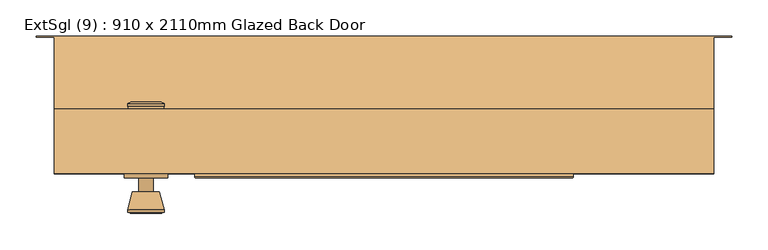
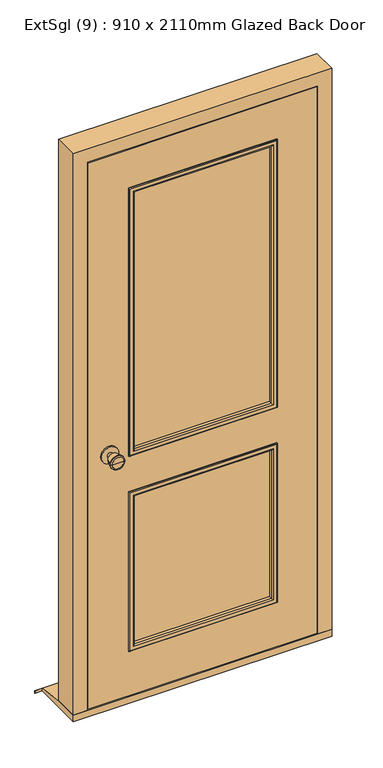
"""IFC4 building model written with IfcOpenShell, lengths in millimetres: door geometry, ExtSgl (9) : 910 x 2110mm Glazed Back Door."""

from ifc_helpers import new_model, si_unit, point, frame, frame_2d, origin, place, context, project, spatial, polyline, circle_curve, ellipse_curve, trimmed, segment, composite_curve, outline, extrude, faceted_brep, source, transform, mapped, element, save
from ifc_brep_helpers import plane_surface, cylinder_surface, revolved_surface, advanced_brep


def extsgl_9_910_x_2110mm_glazed_back_door_d686a627(model_context):
    return source(origin(), model_context, "Body", "SolidModel", [
        advanced_brep(
        [(-328.5, -28.75, 950.0), (-318.5, -28.75, 950.0), (-338.5, -28.75, 950.0), (-308.0241324, -77.75, 950.0), (-328.5, -77.75, 950.0), (-348.9758676, -77.75, 950.0), (-303.5, -75.9221319, 950.0), (-353.5, -75.9221319, 950.0), (-303.5, -72.4584537, 950.0), (-353.5, -72.4584537, 950.0), (-309.863764, -47.75, 950.0), (-347.136236, -47.75, 950.0), (-318.5, -47.75, 950.0), (-338.5, -47.75, 950.0)],
        [
            (0, 1),
            (1, 2, circle_curve(frame((-328.5, -28.75, 950.0), z_axis=(0.0, 1.0, 0.0), x_axis=(-1.0, 0.0, 0.0)), 10.0)),
            (2, 0),
            (2, 1, circle_curve(frame((-328.5, -28.75, 950.0), z_axis=(0.0, 1.0, 0.0), x_axis=(-1.0, 0.0, 0.0)), 10.0)),
            (3, 4),
            (4, 5),
            (5, 3, circle_curve(frame((-328.5, -77.75, 950.0), z_axis=(0.0, -1.0, 0.0), x_axis=(-1.0, 0.0, 0.0)), 20.4758676)),
            (3, 5, circle_curve(frame((-328.5, -77.75, 950.0), z_axis=(0.0, -1.0, 0.0), x_axis=(-1.0, 0.0, 0.0)), 20.4758676)),
            (6, 3),
            (5, 7),
            (7, 6, circle_curve(frame((-328.5, -75.9221319, 950.0), z_axis=(0.0, -1.0, 0.0), x_axis=(-1.0, 0.0, 0.0)), 25.0)),
            (6, 7, circle_curve(frame((-328.5, -75.9221319, 950.0), z_axis=(0.0, -1.0, 0.0), x_axis=(-1.0, 0.0, 0.0)), 25.0)),
            (8, 6),
            (7, 9),
            (9, 8, circle_curve(frame((-328.5, -72.4584537, 950.0), z_axis=(0.0, -1.0, 0.0), x_axis=(-1.0, 0.0, 0.0)), 25.0)),
            (8, 9, circle_curve(frame((-328.5, -72.4584537, 950.0), z_axis=(0.0, -1.0, 0.0), x_axis=(-1.0, 0.0, 0.0)), 25.0)),
            (10, 8),
            (9, 11),
            (11, 10, circle_curve(frame((-328.5, -47.75, 950.0), z_axis=(0.0, -1.0, 0.0), x_axis=(-1.0, 0.0, 0.0)), 18.636236)),
            (10, 11, circle_curve(frame((-328.5, -47.75, 950.0), z_axis=(0.0, -1.0, 0.0), x_axis=(-1.0, 0.0, 0.0)), 18.636236)),
            (12, 10),
            (11, 13),
            (13, 12, circle_curve(frame((-328.5, -47.75, 950.0), z_axis=(0.0, -1.0, 0.0), x_axis=(-1.0, 0.0, 0.0)), 10.0)),
            (12, 13, circle_curve(frame((-328.5, -47.75, 950.0), z_axis=(0.0, -1.0, 0.0), x_axis=(-1.0, 0.0, 0.0)), 10.0)),
            (1, 12),
            (13, 2),
        ],
        [
            plane_surface(frame((-328.5, -28.75, 950.0), z_axis=(0.0, 1.0, 0.0), x_axis=(-1.0, 0.0, 0.0))),
            plane_surface(frame((-328.5, -77.75, 950.0), z_axis=(0.0, -1.0, 0.0), x_axis=(-1.0, 0.0, 0.0))),
            revolved_surface(polyline([(-348.9758676, -77.75, 950.0), (-353.5, -75.9221319, 950.0)]), (-328.5, -28.75, 950.0), (0.0, 1.0, 0.0)),
            cylinder_surface(frame((-328.5, -28.75, 950.0), z_axis=(0.0, 1.0, 0.0), x_axis=(-1.0, 0.0, 0.0)), 25.0),
            revolved_surface(polyline([(-353.5, -72.4584537, 950.0), (-347.136236, -47.75, 950.0)]), (-328.5, -28.75, 950.0), (0.0, 1.0, 0.0)),
            plane_surface(frame((-328.5, -47.75, 950.0), z_axis=(0.0, 1.0, 0.0), x_axis=(-1.0, 0.0, 0.0))),
            cylinder_surface(frame((-328.5, -28.75, 950.0), z_axis=(0.0, 1.0, 0.0), x_axis=(-1.0, 0.0, 0.0)), 10.0),
        ],
        [
            (0, [[1, 2, 3]]),
            (0, [[-3, 4, -1]]),
            (1, [[5, 6, 7]]),
            (1, [[-6, -5, 8]]),
            (2, [[9, -7, 10, 11]]),
            (2, [[-10, -8, -9, 12]]),
            (3, [[13, -11, 14, 15]]),
            (3, [[-14, -12, -13, 16]]),
            (4, [[17, -15, 18, 19]]),
            (4, [[-18, -16, -17, 20]]),
            (5, [[21, -19, 22, 23]]),
            (5, [[-22, -20, -21, 24]]),
            (6, [[25, -23, 26, -2]]),
            (6, [[-26, -24, -25, -4]]),
        ],
    ),
        extrude(outline(composite_curve([segment(trimmed(circle_curve(frame_2d((950.0, -328.5)), 30.0), [point((950.0, -358.5))], [point((950.0, -298.5))], False, "CARTESIAN"), True, "CONTINUOUS"), segment(trimmed(circle_curve(frame_2d((950.0, -328.5)), 30.0), [point((950.0, -298.5))], [point((950.0, -358.5))], False, "CARTESIAN"), True, "CONTINUOUS")], self_intersect=False)), frame((0.0, -28.75, 0.0), z_axis=(0.0, 1.0, 0.0), x_axis=(0.0, 0.0, 1.0)), (0.0, 0.0, 1.0), 6.0),
        advanced_brep(
        [(-328.5, 27.25, 950.0), (-338.5, 27.25, 950.0), (-318.5, 27.25, 950.0), (-308.0241324, 76.25, 950.0), (-348.9758676, 76.25, 950.0), (-328.5, 76.25, 950.0), (-303.5, 74.4221319, 950.0), (-353.5, 74.4221319, 950.0), (-303.5, 70.9584537, 950.0), (-353.5, 70.9584537, 950.0), (-309.863764, 46.25, 950.0), (-347.136236, 46.25, 950.0), (-318.5, 46.25, 950.0), (-338.5, 46.25, 950.0)],
        [
            (0, 1),
            (1, 2, circle_curve(frame((-328.5, 27.25, 950.0), z_axis=(0.0, -1.0, 0.0), x_axis=(-1.0, 0.0, 0.0)), 10.0)),
            (2, 0),
            (2, 1, circle_curve(frame((-328.5, 27.25, 950.0), z_axis=(0.0, -1.0, 0.0), x_axis=(-1.0, 0.0, 0.0)), 10.0)),
            (3, 4, circle_curve(frame((-328.5, 76.25, 950.0), z_axis=(0.0, 1.0, 0.0), x_axis=(-1.0, 0.0, 0.0)), 20.4758676)),
            (4, 5),
            (5, 3),
            (4, 3, circle_curve(frame((-328.5, 76.25, 950.0), z_axis=(0.0, 1.0, 0.0), x_axis=(-1.0, 0.0, 0.0)), 20.4758676)),
            (6, 7, circle_curve(frame((-328.5, 74.4221319, 950.0), z_axis=(0.0, 1.0, 0.0), x_axis=(-1.0, 0.0, 0.0)), 25.0)),
            (7, 4),
            (3, 6),
            (7, 6, circle_curve(frame((-328.5, 74.4221319, 950.0), z_axis=(0.0, 1.0, 0.0), x_axis=(-1.0, 0.0, 0.0)), 25.0)),
            (8, 9, circle_curve(frame((-328.5, 70.9584537, 950.0), z_axis=(0.0, 1.0, 0.0), x_axis=(-1.0, 0.0, 0.0)), 25.0)),
            (9, 7),
            (6, 8),
            (9, 8, circle_curve(frame((-328.5, 70.9584537, 950.0), z_axis=(0.0, 1.0, 0.0), x_axis=(-1.0, 0.0, 0.0)), 25.0)),
            (10, 11, circle_curve(frame((-328.5, 46.25, 950.0), z_axis=(0.0, 1.0, 0.0), x_axis=(-1.0, 0.0, 0.0)), 18.636236)),
            (11, 9),
            (8, 10),
            (11, 10, circle_curve(frame((-328.5, 46.25, 950.0), z_axis=(0.0, 1.0, 0.0), x_axis=(-1.0, 0.0, 0.0)), 18.636236)),
            (12, 13, circle_curve(frame((-328.5, 46.25, 950.0), z_axis=(0.0, 1.0, 0.0), x_axis=(-1.0, 0.0, 0.0)), 10.0)),
            (13, 11),
            (10, 12),
            (13, 12, circle_curve(frame((-328.5, 46.25, 950.0), z_axis=(0.0, 1.0, 0.0), x_axis=(-1.0, 0.0, 0.0)), 10.0)),
            (1, 13),
            (12, 2),
        ],
        [
            plane_surface(frame((-328.5, 27.25, 950.0), z_axis=(0.0, -1.0, 0.0), x_axis=(-1.0, 0.0, 0.0))),
            plane_surface(frame((-328.5, 76.25, 950.0), z_axis=(0.0, 1.0, 0.0), x_axis=(-1.0, 0.0, 0.0))),
            revolved_surface(polyline([(-348.9758676, 76.25, 950.0), (-353.5, 74.4221319, 950.0)]), (-328.5, 27.25, 950.0), (0.0, -1.0, 0.0)),
            cylinder_surface(frame((-328.5, 27.25, 950.0), z_axis=(0.0, -1.0, 0.0), x_axis=(-1.0, 0.0, 0.0)), 25.0),
            revolved_surface(polyline([(-353.5, 70.9584537, 950.0), (-347.136236, 46.25, 950.0)]), (-328.5, 27.25, 950.0), (0.0, -1.0, 0.0)),
            plane_surface(frame((-328.5, 46.25, 950.0), z_axis=(0.0, -1.0, 0.0), x_axis=(-1.0, 0.0, 0.0))),
            cylinder_surface(frame((-328.5, 27.25, 950.0), z_axis=(0.0, -1.0, 0.0), x_axis=(-1.0, 0.0, 0.0)), 10.0),
        ],
        [
            (0, [[1, 2, 3]]),
            (0, [[-3, 4, -1]]),
            (1, [[5, 6, 7]]),
            (1, [[8, -7, -6]]),
            (2, [[9, 10, -5, 11]]),
            (2, [[12, -11, -8, -10]]),
            (3, [[13, 14, -9, 15]]),
            (3, [[16, -15, -12, -14]]),
            (4, [[17, 18, -13, 19]]),
            (4, [[20, -19, -16, -18]]),
            (5, [[21, 22, -17, 23]]),
            (5, [[24, -23, -20, -22]]),
            (6, [[-2, 25, -21, 26]]),
            (6, [[-4, -26, -24, -25]]),
        ],
    ),
        extrude(outline(composite_curve([segment(trimmed(circle_curve(frame_2d((950.0, -328.5)), 30.0), [point((950.0, -358.5))], [point((950.0, -298.5))], False, "CARTESIAN"), True, "CONTINUOUS"), segment(trimmed(circle_curve(frame_2d((950.0, -328.5)), 30.0), [point((950.0, -298.5))], [point((950.0, -358.5))], False, "CARTESIAN"), True, "CONTINUOUS")], self_intersect=False)), frame((0.0, 21.25, 0.0), z_axis=(0.0, 1.0, 0.0), x_axis=(0.0, 0.0, 1.0)), (0.0, 0.0, 1.0), 6.0),
        faceted_brep([(384.5, 66.25, 25.0), (455.0, 66.25, 25.0), (455.0, -22.75, 25.0), (406.5, -22.75, 25.0), (406.5, 24.25, 25.0), (384.5, 24.25, 25.0), (384.5, 66.25, 2039.5), (-384.5, 66.25, 2039.5), (-384.5, 66.25, 25.0), (-455.0, 66.25, 25.0), (-455.0, 66.25, 2110.0), (455.0, 66.25, 2110.0), (455.0, -22.75, 2110.0), (-455.0, -22.75, 2110.0), (-455.0, -22.75, 25.0), (-406.5, -22.75, 25.0), (-406.5, -22.75, 2061.5), (406.5, -22.75, 2061.5), (406.5, 24.25, 2061.5), (-406.5, 24.25, 2061.5), (-406.5, 24.25, 25.0), (-384.5, 24.25, 25.0), (-384.5, 24.25, 2039.5), (384.5, 24.25, 2039.5)], [[[0, 1, 2, 3, 4, 5]], [[1, 0, 6, 7, 8, 9, 10, 11]], [[2, 1, 11, 12]], [[3, 2, 12, 13, 14, 15, 16, 17]], [[4, 3, 17, 18]], [[5, 4, 18, 19, 20, 21, 22, 23]], [[0, 5, 23, 6]], [[7, 22, 21, 8]], [[8, 21, 20, 15, 14, 9]], [[13, 10, 9, 14]], [[19, 16, 15, 20]], [[12, 11, 10, 13]], [[18, 17, 16, 19]], [[6, 23, 22, 7]]]),
        extrude(outline(polyline([(253.5, -12.75), (-253.5, -12.75), (-253.5, 11.25), (253.5, 11.25), (253.5, -12.75)])), frame((0.0, 0.0, 204.0), z_axis=(0.0, 0.0, 1.0), x_axis=(1.0, 0.0, 0.0)), (0.0, 0.0, 1.0), 575.0),
        extrude(outline(polyline([(253.5, -12.75), (-253.5, -12.75), (-253.5, 11.25), (253.5, 11.25), (253.5, -12.75)])), frame((0.0, 0.0, 929.0), z_axis=(0.0, 0.0, 1.0), x_axis=(1.0, 0.0, 0.0)), (0.0, 0.0, 1.0), 979.5),
        faceted_brep([(480.0, 167.25, 0.0), (480.0, 167.25, 9.0947221), (480.0, 166.25, 9.2522001), (480.0, 166.25, 0.0), (-480.0, 167.25, 9.0947221), (-480.0, 167.25, 0.0), (-480.0, 166.25, 0.0), (-480.0, 166.25, 9.2522001), (455.0, 166.25, 0.0), (455.0, -22.75, 0.0), (-455.0, -22.75, 0.0), (-455.0, 166.25, 0.0), (-455.0, 166.25, 9.2522001), (-455.0, 66.25, 25.0), (455.0, 66.25, 25.0), (455.0, 166.25, 9.2522001), (-455.0, -22.75, 25.0), (455.0, -22.75, 25.0)], [[[0, 1, 2, 3]], [[4, 5, 6, 7]], [[5, 0, 3, 8, 9, 10, 11, 6]], [[1, 0, 5, 4]], [[1, 4, 7, 12, 13, 14, 15, 2]], [[13, 16, 17, 14]], [[16, 10, 9, 17]], [[12, 11, 10, 16, 13]], [[11, 12, 7, 6]], [[8, 15, 14, 17, 9]], [[15, 8, 3, 2]]]),
        extrude(outline(polyline([(29.0, 403.5), (2058.5, 403.5), (2058.5, -404.4250294), (29.0, -404.4250294), (29.0, 403.5)]), holes=[polyline([(929.0, -253.5), (1908.5, -253.5), (1908.5, 253.5), (929.0, 253.5), (929.0, -253.5)]), polyline([(204.0, -253.5), (779.0, -253.5), (779.0, 253.5), (204.0, 253.5), (204.0, -253.5)])]), frame((0.0, -22.75, 0.0), z_axis=(0.0, 1.0, 0.0), x_axis=(0.0, 0.0, 1.0)), (0.0, 0.0, 1.0), 44.0),
        advanced_brep(
        [(253.5, -12.75, 779.0), (253.5, -22.75, 779.0), (253.5, -22.75, 204.0), (253.5, -12.75, 204.0), (241.5, -23.75, 767.0), (241.5, -12.75, 767.0), (241.5, -12.75, 216.0), (241.5, -23.75, 216.0), (246.5, -28.75, 772.0), (246.5, -28.75, 211.0), (261.5, -26.75, 787.0), (259.5, -28.75, 785.0), (259.5, -28.75, 198.0), (261.5, -26.75, 196.0), (261.5, -22.75, 787.0), (261.5, -22.75, 196.0), (-253.5, -22.75, 204.0), (-253.5, -12.75, 204.0), (-241.5, -12.75, 216.0), (-241.5, -23.75, 216.0), (-246.5, -28.75, 211.0), (-259.5, -28.75, 198.0), (-261.5, -26.75, 196.0), (-261.5, -22.75, 196.0), (-253.5, -22.75, 779.0), (-253.5, -12.75, 779.0), (-241.5, -12.75, 767.0), (-241.5, -23.75, 767.0), (-246.5, -28.75, 772.0), (-259.5, -28.75, 785.0), (-261.5, -26.75, 787.0), (-261.5, -22.75, 787.0)],
        [
            (0, 1),
            (1, 2),
            (2, 3),
            (3, 0),
            (4, 5),
            (5, 6),
            (6, 7),
            (7, 4),
            (8, 4, ellipse_curve(frame((246.5, -23.75, 772.0), z_axis=(0.7071067811865521, 0.0, -0.7071067811865428), x_axis=(0.7071067811865428, 0.0, 0.7071067811865522)), 7.0710678, 5.0)),
            (7, 9, ellipse_curve(frame((246.5, -23.75, 211.0), z_axis=(0.7071067811865428, 0.0, 0.7071067811865521), x_axis=(-0.707106781186552, 0.0, 0.7071067811865429)), 7.0710678, 5.0)),
            (9, 8),
            (10, 11, ellipse_curve(frame((259.5, -26.75, 785.0), z_axis=(0.7071067811865521, 0.0, -0.7071067811865428), x_axis=(0.7071067811865428, 0.0, 0.7071067811865522)), 2.8284271, 2.0)),
            (11, 12),
            (12, 13, ellipse_curve(frame((259.5, -26.75, 198.0), z_axis=(0.7071067811865428, 0.0, 0.7071067811865521), x_axis=(-0.707106781186552, 0.0, 0.7071067811865429)), 2.8284271, 2.0)),
            (13, 10),
            (14, 10),
            (13, 15),
            (15, 14),
            (2, 16),
            (16, 17),
            (17, 3),
            (6, 18),
            (18, 19),
            (19, 7),
            (19, 20, ellipse_curve(frame((-246.5, -23.75, 211.0), z_axis=(0.7071067811865521, 0.0, -0.7071067811865428), x_axis=(0.7071067811865429, 0.0, 0.707106781186552)), 7.0710678, 5.0)),
            (20, 9),
            (12, 21),
            (21, 22, ellipse_curve(frame((-259.5, -26.75, 198.0), z_axis=(0.7071067811865521, 0.0, -0.7071067811865428), x_axis=(0.7071067811865429, 0.0, 0.707106781186552)), 2.8284271, 2.0)),
            (22, 13),
            (22, 23),
            (23, 15),
            (16, 24),
            (24, 25),
            (25, 17),
            (18, 26),
            (26, 27),
            (27, 19),
            (27, 28, ellipse_curve(frame((-246.5, -23.75, 772.0), z_axis=(-0.7071067811865428, 0.0, -0.7071067811865521), x_axis=(0.707106781186552, 0.0, -0.707106781186543)), 7.0710678, 5.0)),
            (28, 20),
            (21, 29),
            (29, 30, ellipse_curve(frame((-259.5, -26.75, 785.0), z_axis=(-0.7071067811865428, 0.0, -0.7071067811865521), x_axis=(0.707106781186552, 0.0, -0.707106781186543)), 2.8284271, 2.0)),
            (30, 22),
            (30, 31),
            (31, 23),
            (31, 14),
            (1, 24),
            (0, 25),
            (5, 26),
            (4, 27),
            (8, 28),
            (11, 29),
            (10, 30),
        ],
        [
            plane_surface(frame((253.5, -22.75, 779.0), z_axis=(1.0, 0.0, 0.0), x_axis=(0.0, 0.0, -1.0))),
            plane_surface(frame((241.5, -12.75, 767.0), z_axis=(-1.0, 0.0, 0.0), x_axis=(0.0, 0.0, -1.0))),
            cylinder_surface(frame((246.5, -23.75, 779.0), z_axis=(0.0, 0.0, 1.0), x_axis=(1.0, 0.0, 0.0)), 5.0),
            cylinder_surface(frame((259.5, -26.75, 779.0), z_axis=(0.0, 0.0, 1.0), x_axis=(1.0, 0.0, 0.0)), 2.0),
            plane_surface(frame((261.5, -26.75, 787.0), z_axis=(1.0, 0.0, 0.0), x_axis=(0.0, 0.0, -1.0))),
            plane_surface(frame((253.5, -22.75, 204.0), z_axis=(0.0, 0.0, -1.0), x_axis=(-1.0, 0.0, 0.0))),
            plane_surface(frame((241.5, -12.75, 216.0), z_axis=(0.0, 0.0, 1.0), x_axis=(-1.0, 0.0, 0.0))),
            cylinder_surface(frame((253.5, -23.75, 211.0), z_axis=(1.0, 0.0, 0.0), x_axis=(0.0, 0.0, -1.0)), 5.0),
            cylinder_surface(frame((253.5, -26.75, 198.0), z_axis=(1.0, 0.0, 0.0), x_axis=(0.0, 0.0, -1.0)), 2.0),
            plane_surface(frame((261.5, -26.75, 196.0), z_axis=(0.0, 0.0, -1.0), x_axis=(-1.0, 0.0, 0.0))),
            plane_surface(frame((-253.5, -22.75, 204.0), z_axis=(-1.0, 0.0, 0.0), x_axis=(0.0, 0.0, 1.0))),
            plane_surface(frame((-241.5, -12.75, 216.0), z_axis=(1.0, 0.0, 0.0), x_axis=(0.0, 0.0, 1.0))),
            cylinder_surface(frame((-246.5, -23.75, 204.0), z_axis=(0.0, 0.0, -1.0), x_axis=(-1.0, 0.0, 0.0)), 5.0),
            cylinder_surface(frame((-259.5, -26.75, 204.0), z_axis=(0.0, 0.0, -1.0), x_axis=(-1.0, 0.0, 0.0)), 2.0),
            plane_surface(frame((-261.5, -26.75, 196.0), z_axis=(-1.0, 0.0, 0.0), x_axis=(0.0, 0.0, 1.0))),
            plane_surface(frame((-261.5, -22.75, 787.0), z_axis=(0.0, 1.0, 0.0), x_axis=(1.0, 0.0, 0.0))),
            plane_surface(frame((-253.5, -22.75, 779.0), z_axis=(0.0, 0.0, 1.0), x_axis=(1.0, 0.0, 0.0))),
            plane_surface(frame((-253.5, -12.75, 779.0), z_axis=(0.0, 1.0, 0.0), x_axis=(1.0, 0.0, 0.0))),
            plane_surface(frame((-241.5, -12.75, 767.0), z_axis=(0.0, 0.0, -1.0), x_axis=(1.0, 0.0, 0.0))),
            cylinder_surface(frame((-253.5, -23.75, 772.0), z_axis=(-1.0, 0.0, 0.0), x_axis=(0.0, 0.0, 1.0)), 5.0),
            plane_surface(frame((-246.5, -28.75, 772.0), z_axis=(0.0, -1.0, 0.0), x_axis=(1.0, 0.0, 0.0))),
            cylinder_surface(frame((-253.5, -26.75, 785.0), z_axis=(-1.0, 0.0, 0.0), x_axis=(0.0, 0.0, 1.0)), 2.0),
            plane_surface(frame((-261.5, -26.75, 787.0), z_axis=(0.0, 0.0, 1.0), x_axis=(1.0, 0.0, 0.0))),
        ],
        [
            (0, [[1, 2, 3, 4]]),
            (1, [[5, 6, 7, 8]]),
            (2, [[9, -8, 10, 11]]),
            (3, [[12, 13, 14, 15]]),
            (4, [[16, -15, 17, 18]]),
            (5, [[-3, 19, 20, 21]]),
            (6, [[-7, 22, 23, 24]]),
            (7, [[-10, -24, 25, 26]]),
            (8, [[-14, 27, 28, 29]]),
            (9, [[-17, -29, 30, 31]]),
            (10, [[-20, 32, 33, 34]]),
            (11, [[-23, 35, 36, 37]]),
            (12, [[-25, -37, 38, 39]]),
            (13, [[-28, 40, 41, 42]]),
            (14, [[-30, -42, 43, 44]]),
            (15, [[-31, -44, 45, -18], [46, -32, -19, -2]]),
            (16, [[-33, -46, -1, 47]]),
            (17, [[-21, -34, -47, -4], [48, -35, -22, -6]]),
            (18, [[-36, -48, -5, 49]]),
            (19, [[-38, -49, -9, 50]]),
            (20, [[51, -40, -27, -13], [-26, -39, -50, -11]]),
            (21, [[-41, -51, -12, 52]]),
            (22, [[-43, -52, -16, -45]]),
        ],
    ),
        advanced_brep(
        [(-261.5, 25.25, 196.0), (-261.5, 21.25, 196.0), (-261.5, 21.25, 787.0), (-261.5, 25.25, 787.0), (-259.5, 27.25, 198.0), (-259.5, 27.25, 785.0), (-241.5, 22.25, 216.0), (-246.5, 27.25, 211.0), (-246.5, 27.25, 772.0), (-241.5, 22.25, 767.0), (-241.5, 11.25, 216.0), (-241.5, 11.25, 767.0), (-253.5, 21.25, 204.0), (-253.5, 11.25, 204.0), (-253.5, 11.25, 779.0), (-253.5, 21.25, 779.0), (261.5, 21.25, 787.0), (261.5, 25.25, 787.0), (259.5, 27.25, 785.0), (246.5, 27.25, 772.0), (241.5, 22.25, 767.0), (241.5, 11.25, 767.0), (253.5, 11.25, 779.0), (253.5, 21.25, 779.0), (261.5, 21.25, 196.0), (261.5, 25.25, 196.0), (259.5, 27.25, 198.0), (246.5, 27.25, 211.0), (241.5, 22.25, 216.0), (241.5, 11.25, 216.0), (253.5, 11.25, 204.0), (253.5, 21.25, 204.0)],
        [
            (0, 1),
            (1, 2),
            (2, 3),
            (3, 0),
            (4, 0, ellipse_curve(frame((-259.5, 25.25, 198.0), z_axis=(-0.7071067811865475, 0.0, 0.7071067811865475), x_axis=(-0.7071067811865474, 0.0, -0.7071067811865476)), 2.8284271, 2.0)),
            (3, 5, ellipse_curve(frame((-259.5, 25.25, 785.0), z_axis=(-0.7071067811865475, 0.0, -0.7071067811865475), x_axis=(0.7071067811865474, 0.0, -0.7071067811865476)), 2.8284271, 2.0)),
            (5, 4),
            (6, 7, ellipse_curve(frame((-246.5, 22.25, 211.0), z_axis=(-0.7071067811865475, 0.0, 0.7071067811865475), x_axis=(-0.7071067811865474, 0.0, -0.7071067811865476)), 7.0710678, 5.0)),
            (7, 8),
            (8, 9, ellipse_curve(frame((-246.5, 22.25, 772.0), z_axis=(-0.7071067811865475, 0.0, -0.7071067811865475), x_axis=(0.7071067811865474, 0.0, -0.7071067811865476)), 7.0710678, 5.0)),
            (9, 6),
            (10, 6),
            (9, 11),
            (11, 10),
            (12, 13),
            (13, 14),
            (14, 15),
            (15, 12),
            (2, 16),
            (16, 17),
            (17, 3),
            (17, 18, ellipse_curve(frame((259.5, 25.25, 785.0), z_axis=(-0.7071067811865475, 0.0, 0.7071067811865475), x_axis=(-0.7071067811865476, 0.0, -0.7071067811865474)), 2.8284271, 2.0)),
            (18, 5),
            (8, 19),
            (19, 20, ellipse_curve(frame((246.5, 22.25, 772.0), z_axis=(-0.7071067811865475, 0.0, 0.7071067811865475), x_axis=(-0.7071067811865476, 0.0, -0.7071067811865474)), 7.0710678, 5.0)),
            (20, 9),
            (20, 21),
            (21, 11),
            (14, 22),
            (22, 23),
            (23, 15),
            (16, 24),
            (24, 25),
            (25, 17),
            (25, 26, ellipse_curve(frame((259.5, 25.25, 198.0), z_axis=(0.7071067811865475, 0.0, 0.7071067811865475), x_axis=(-0.7071067811865474, 0.0, 0.7071067811865476)), 2.8284271, 2.0)),
            (26, 18),
            (19, 27),
            (27, 28, ellipse_curve(frame((246.5, 22.25, 211.0), z_axis=(0.7071067811865475, 0.0, 0.7071067811865475), x_axis=(-0.7071067811865474, 0.0, 0.7071067811865476)), 7.0710678, 5.0)),
            (28, 20),
            (28, 29),
            (29, 21),
            (22, 30),
            (30, 31),
            (31, 23),
            (24, 1),
            (0, 25),
            (4, 26),
            (7, 27),
            (6, 28),
            (10, 29),
            (13, 30),
            (12, 31),
        ],
        [
            plane_surface(frame((-261.5, 21.25, 196.0), z_axis=(-1.0, 0.0, 0.0), x_axis=(0.0, 0.0, 1.0))),
            cylinder_surface(frame((-259.5, 25.25, 204.0), z_axis=(0.0, 0.0, -1.0), x_axis=(-1.0, 0.0, 0.0)), 2.0),
            cylinder_surface(frame((-246.5, 22.25, 204.0), z_axis=(0.0, 0.0, -1.0), x_axis=(-1.0, 0.0, 0.0)), 5.0),
            plane_surface(frame((-241.5, 22.25, 216.0), z_axis=(1.0, 0.0, 0.0), x_axis=(0.0, 0.0, 1.0))),
            plane_surface(frame((-253.5, 11.25, 204.0), z_axis=(-1.0, 0.0, 0.0), x_axis=(0.0, 0.0, 1.0))),
            plane_surface(frame((-261.5, 21.25, 787.0), z_axis=(0.0, 0.0, 1.0), x_axis=(1.0, 0.0, 0.0))),
            cylinder_surface(frame((-253.5, 25.25, 785.0), z_axis=(-1.0, 0.0, 0.0), x_axis=(0.0, 0.0, 1.0)), 2.0),
            cylinder_surface(frame((-253.5, 22.25, 772.0), z_axis=(-1.0, 0.0, 0.0), x_axis=(0.0, 0.0, 1.0)), 5.0),
            plane_surface(frame((-241.5, 22.25, 767.0), z_axis=(0.0, 0.0, -1.0), x_axis=(1.0, 0.0, 0.0))),
            plane_surface(frame((-253.5, 11.25, 779.0), z_axis=(0.0, 0.0, 1.0), x_axis=(1.0, 0.0, 0.0))),
            plane_surface(frame((261.5, 21.25, 787.0), z_axis=(1.0, 0.0, 0.0), x_axis=(0.0, 0.0, -1.0))),
            cylinder_surface(frame((259.5, 25.25, 779.0), z_axis=(0.0, 0.0, 1.0), x_axis=(1.0, 0.0, 0.0)), 2.0),
            cylinder_surface(frame((246.5, 22.25, 779.0), z_axis=(0.0, 0.0, 1.0), x_axis=(1.0, 0.0, 0.0)), 5.0),
            plane_surface(frame((241.5, 22.25, 767.0), z_axis=(-1.0, 0.0, 0.0), x_axis=(0.0, 0.0, -1.0))),
            plane_surface(frame((253.5, 11.25, 779.0), z_axis=(1.0, 0.0, 0.0), x_axis=(0.0, 0.0, -1.0))),
            plane_surface(frame((261.5, 21.25, 196.0), z_axis=(0.0, 0.0, -1.0), x_axis=(-1.0, 0.0, 0.0))),
            cylinder_surface(frame((253.5, 25.25, 198.0), z_axis=(1.0, 0.0, 0.0), x_axis=(0.0, 0.0, -1.0)), 2.0),
            plane_surface(frame((259.5, 27.25, 198.0), z_axis=(0.0, 1.0, 0.0), x_axis=(-1.0, 0.0, 0.0))),
            cylinder_surface(frame((253.5, 22.25, 211.0), z_axis=(1.0, 0.0, 0.0), x_axis=(0.0, 0.0, -1.0)), 5.0),
            plane_surface(frame((241.5, 22.25, 216.0), z_axis=(0.0, 0.0, 1.0), x_axis=(-1.0, 0.0, 0.0))),
            plane_surface(frame((241.5, 11.25, 216.0), z_axis=(0.0, -1.0, 0.0), x_axis=(-1.0, 0.0, 0.0))),
            plane_surface(frame((253.5, 11.25, 204.0), z_axis=(0.0, 0.0, -1.0), x_axis=(-1.0, 0.0, 0.0))),
            plane_surface(frame((253.5, 21.25, 204.0), z_axis=(0.0, -1.0, 0.0), x_axis=(-1.0, 0.0, 0.0))),
        ],
        [
            (0, [[1, 2, 3, 4]]),
            (1, [[5, -4, 6, 7]]),
            (2, [[8, 9, 10, 11]]),
            (3, [[12, -11, 13, 14]]),
            (4, [[15, 16, 17, 18]]),
            (5, [[-3, 19, 20, 21]]),
            (6, [[-6, -21, 22, 23]]),
            (7, [[-10, 24, 25, 26]]),
            (8, [[-13, -26, 27, 28]]),
            (9, [[-17, 29, 30, 31]]),
            (10, [[-20, 32, 33, 34]]),
            (11, [[-22, -34, 35, 36]]),
            (12, [[-25, 37, 38, 39]]),
            (13, [[-27, -39, 40, 41]]),
            (14, [[-30, 42, 43, 44]]),
            (15, [[-33, 45, -1, 46]]),
            (16, [[-35, -46, -5, 47]]),
            (17, [[-23, -36, -47, -7], [48, -37, -24, -9]]),
            (18, [[-38, -48, -8, 49]]),
            (19, [[-40, -49, -12, 50]]),
            (20, [[51, -42, -29, -16], [-28, -41, -50, -14]]),
            (21, [[-43, -51, -15, 52]]),
            (22, [[-45, -32, -19, -2], [-31, -44, -52, -18]]),
        ],
    ),
        advanced_brep(
        [(261.5, -26.75, 921.0), (261.5, -22.75, 921.0), (261.5, -22.75, 1916.5), (261.5, -26.75, 1916.5), (259.5, -28.75, 923.0), (259.5, -28.75, 1914.5), (241.5, -23.75, 941.0), (246.5, -28.75, 936.0), (246.5, -28.75, 1901.5), (241.5, -23.75, 1896.5), (241.5, -12.75, 941.0), (241.5, -12.75, 1896.5), (253.5, -22.75, 929.0), (253.5, -12.75, 929.0), (253.5, -12.75, 1908.5), (253.5, -22.75, 1908.5), (-261.5, -22.75, 1916.5), (-261.5, -26.75, 1916.5), (-259.5, -28.75, 1914.5), (-246.5, -28.75, 1901.5), (-241.5, -23.75, 1896.5), (-241.5, -12.75, 1896.5), (-253.5, -12.75, 1908.5), (-253.5, -22.75, 1908.5), (-261.5, -22.75, 921.0), (-261.5, -26.75, 921.0), (-259.5, -28.75, 923.0), (-246.5, -28.75, 936.0), (-241.5, -23.75, 941.0), (-241.5, -12.75, 941.0), (-253.5, -12.75, 929.0), (-253.5, -22.75, 929.0)],
        [
            (0, 1),
            (1, 2),
            (2, 3),
            (3, 0),
            (4, 0, ellipse_curve(frame((259.5, -26.75, 923.0), z_axis=(0.7071067811865429, 0.0, 0.707106781186552), x_axis=(0.7071067811865518, 0.0, -0.7071067811865431)), 2.8284271, 2.0)),
            (3, 5, ellipse_curve(frame((259.5, -26.75, 1914.5), z_axis=(0.707106781186552, 0.0, -0.7071067811865429), x_axis=(-0.7071067811865428, 0.0, -0.7071067811865521)), 2.8284271, 2.0)),
            (5, 4),
            (6, 7, ellipse_curve(frame((246.5, -23.75, 936.0), z_axis=(0.7071067811865429, 0.0, 0.707106781186552), x_axis=(0.7071067811865518, 0.0, -0.7071067811865431)), 7.0710678, 5.0)),
            (7, 8),
            (8, 9, ellipse_curve(frame((246.5, -23.75, 1901.5), z_axis=(0.707106781186552, 0.0, -0.7071067811865429), x_axis=(-0.7071067811865428, 0.0, -0.7071067811865521)), 7.0710678, 5.0)),
            (9, 6),
            (10, 6),
            (9, 11),
            (11, 10),
            (12, 13),
            (13, 14),
            (14, 15),
            (15, 12),
            (2, 16),
            (16, 17),
            (17, 3),
            (17, 18, ellipse_curve(frame((-259.5, -26.75, 1914.5), z_axis=(0.7071067811865429, 0.0, 0.7071067811865521), x_axis=(0.7071067811865521, 0.0, -0.7071067811865429)), 2.8284271, 2.0)),
            (18, 5),
            (8, 19),
            (19, 20, ellipse_curve(frame((-246.5, -23.75, 1901.5), z_axis=(0.7071067811865429, 0.0, 0.7071067811865521), x_axis=(0.7071067811865521, 0.0, -0.7071067811865429)), 7.0710678, 5.0)),
            (20, 9),
            (20, 21),
            (21, 11),
            (14, 22),
            (22, 23),
            (23, 15),
            (16, 24),
            (24, 25),
            (25, 17),
            (25, 26, ellipse_curve(frame((-259.5, -26.75, 923.0), z_axis=(-0.7071067811865521, 0.0, 0.7071067811865429), x_axis=(0.7071067811865429, 0.0, 0.707106781186552)), 2.8284271, 2.0)),
            (26, 18),
            (19, 27),
            (27, 28, ellipse_curve(frame((-246.5, -23.75, 936.0), z_axis=(-0.7071067811865521, 0.0, 0.7071067811865429), x_axis=(0.7071067811865429, 0.0, 0.707106781186552)), 7.0710678, 5.0)),
            (28, 20),
            (28, 29),
            (29, 21),
            (22, 30),
            (30, 31),
            (31, 23),
            (24, 1),
            (0, 25),
            (4, 26),
            (7, 27),
            (6, 28),
            (10, 29),
            (13, 30),
            (12, 31),
        ],
        [
            plane_surface(frame((261.5, -22.75, 921.0), z_axis=(1.0, 0.0, 0.0), x_axis=(0.0, 0.0, 1.0))),
            cylinder_surface(frame((259.5, -26.75, 929.0), z_axis=(0.0, 0.0, -1.0), x_axis=(1.0, 0.0, 0.0)), 2.0),
            cylinder_surface(frame((246.5, -23.75, 929.0), z_axis=(0.0, 0.0, -1.0), x_axis=(1.0, 0.0, 0.0)), 5.0),
            plane_surface(frame((241.5, -23.75, 941.0), z_axis=(-1.0, 0.0, 0.0), x_axis=(0.0, 0.0, 1.0))),
            plane_surface(frame((253.5, -12.75, 929.0), z_axis=(1.0, 0.0, 0.0), x_axis=(0.0, 0.0, 1.0))),
            plane_surface(frame((261.5, -22.75, 1916.5), z_axis=(0.0, 0.0, 1.0), x_axis=(-1.0, 0.0, 0.0))),
            cylinder_surface(frame((253.5, -26.75, 1914.5), z_axis=(1.0, 0.0, 0.0), x_axis=(0.0, 0.0, 1.0)), 2.0),
            cylinder_surface(frame((253.5, -23.75, 1901.5), z_axis=(1.0, 0.0, 0.0), x_axis=(0.0, 0.0, 1.0)), 5.0),
            plane_surface(frame((241.5, -23.75, 1896.5), z_axis=(0.0, 0.0, -1.0), x_axis=(-1.0, 0.0, 0.0))),
            plane_surface(frame((253.5, -12.75, 1908.5), z_axis=(0.0, 0.0, 1.0), x_axis=(-1.0, 0.0, 0.0))),
            plane_surface(frame((-261.5, -22.75, 1916.5), z_axis=(-1.0, 0.0, 0.0), x_axis=(0.0, 0.0, -1.0))),
            cylinder_surface(frame((-259.5, -26.75, 1908.5), z_axis=(0.0, 0.0, 1.0), x_axis=(-1.0, 0.0, 0.0)), 2.0),
            cylinder_surface(frame((-246.5, -23.75, 1908.5), z_axis=(0.0, 0.0, 1.0), x_axis=(-1.0, 0.0, 0.0)), 5.0),
            plane_surface(frame((-241.5, -23.75, 1896.5), z_axis=(1.0, 0.0, 0.0), x_axis=(0.0, 0.0, -1.0))),
            plane_surface(frame((-253.5, -12.75, 1908.5), z_axis=(-1.0, 0.0, 0.0), x_axis=(0.0, 0.0, -1.0))),
            plane_surface(frame((-261.5, -22.75, 921.0), z_axis=(0.0, 0.0, -1.0), x_axis=(1.0, 0.0, 0.0))),
            cylinder_surface(frame((-253.5, -26.75, 923.0), z_axis=(-1.0, 0.0, 0.0), x_axis=(0.0, 0.0, -1.0)), 2.0),
            plane_surface(frame((-259.5, -28.75, 923.0), z_axis=(0.0, -1.0, 0.0), x_axis=(1.0, 0.0, 0.0))),
            cylinder_surface(frame((-253.5, -23.75, 936.0), z_axis=(-1.0, 0.0, 0.0), x_axis=(0.0, 0.0, -1.0)), 5.0),
            plane_surface(frame((-241.5, -23.75, 941.0), z_axis=(0.0, 0.0, 1.0), x_axis=(1.0, 0.0, 0.0))),
            plane_surface(frame((-241.5, -12.75, 941.0), z_axis=(0.0, 1.0, 0.0), x_axis=(1.0, 0.0, 0.0))),
            plane_surface(frame((-253.5, -12.75, 929.0), z_axis=(0.0, 0.0, -1.0), x_axis=(1.0, 0.0, 0.0))),
            plane_surface(frame((-253.5, -22.75, 929.0), z_axis=(0.0, 1.0, 0.0), x_axis=(1.0, 0.0, 0.0))),
        ],
        [
            (0, [[1, 2, 3, 4]]),
            (1, [[5, -4, 6, 7]]),
            (2, [[8, 9, 10, 11]]),
            (3, [[12, -11, 13, 14]]),
            (4, [[15, 16, 17, 18]]),
            (5, [[-3, 19, 20, 21]]),
            (6, [[-6, -21, 22, 23]]),
            (7, [[-10, 24, 25, 26]]),
            (8, [[-13, -26, 27, 28]]),
            (9, [[-17, 29, 30, 31]]),
            (10, [[-20, 32, 33, 34]]),
            (11, [[-22, -34, 35, 36]]),
            (12, [[-25, 37, 38, 39]]),
            (13, [[-27, -39, 40, 41]]),
            (14, [[-30, 42, 43, 44]]),
            (15, [[-33, 45, -1, 46]]),
            (16, [[-35, -46, -5, 47]]),
            (17, [[-23, -36, -47, -7], [48, -37, -24, -9]]),
            (18, [[-38, -48, -8, 49]]),
            (19, [[-40, -49, -12, 50]]),
            (20, [[51, -42, -29, -16], [-28, -41, -50, -14]]),
            (21, [[-43, -51, -15, 52]]),
            (22, [[-45, -32, -19, -2], [-31, -44, -52, -18]]),
        ],
    ),
        advanced_brep(
        [(-261.5, 25.25, 921.0), (-261.5, 21.25, 921.0), (-261.5, 21.25, 1916.5), (-261.5, 25.25, 1916.5), (-259.5, 27.25, 923.0), (-259.5, 27.25, 1914.5), (-241.5, 22.25, 941.0), (-246.5, 27.25, 936.0), (-246.5, 27.25, 1901.5), (-241.5, 22.25, 1896.5), (-241.5, 11.25, 941.0), (-241.5, 11.25, 1896.5), (-253.5, 21.25, 929.0), (-253.5, 11.25, 929.0), (-253.5, 11.25, 1908.5), (-253.5, 21.25, 1908.5), (261.5, 21.25, 1916.5), (261.5, 25.25, 1916.5), (259.5, 27.25, 1914.5), (246.5, 27.25, 1901.5), (241.5, 22.25, 1896.5), (241.5, 11.25, 1896.5), (253.5, 11.25, 1908.5), (253.5, 21.25, 1908.5), (261.5, 21.25, 921.0), (261.5, 25.25, 921.0), (259.5, 27.25, 923.0), (246.5, 27.25, 936.0), (241.5, 22.25, 941.0), (241.5, 11.25, 941.0), (253.5, 11.25, 929.0), (253.5, 21.25, 929.0)],
        [
            (0, 1),
            (1, 2),
            (2, 3),
            (3, 0),
            (4, 0, ellipse_curve(frame((-259.5, 25.25, 923.0), z_axis=(-0.7071067811865474, 0.0, 0.7071067811865476), x_axis=(-0.7071067811865475, 0.0, -0.7071067811865476)), 2.8284271, 2.0)),
            (3, 5, ellipse_curve(frame((-259.5, 25.25, 1914.5), z_axis=(-0.7071067811865476, 0.0, -0.7071067811865474), x_axis=(0.7071067811865474, 0.0, -0.7071067811865478)), 2.8284271, 2.0)),
            (5, 4),
            (6, 7, ellipse_curve(frame((-246.5, 22.25, 936.0), z_axis=(-0.7071067811865474, 0.0, 0.7071067811865476), x_axis=(-0.7071067811865475, 0.0, -0.7071067811865476)), 7.0710678, 5.0)),
            (7, 8),
            (8, 9, ellipse_curve(frame((-246.5, 22.25, 1901.5), z_axis=(-0.7071067811865476, 0.0, -0.7071067811865474), x_axis=(0.7071067811865474, 0.0, -0.7071067811865478)), 7.0710678, 5.0)),
            (9, 6),
            (10, 6),
            (9, 11),
            (11, 10),
            (12, 13),
            (13, 14),
            (14, 15),
            (15, 12),
            (2, 16),
            (16, 17),
            (17, 3),
            (17, 18, ellipse_curve(frame((259.5, 25.25, 1914.5), z_axis=(-0.7071067811865474, 0.0, 0.7071067811865476), x_axis=(-0.7071067811865478, 0.0, -0.7071067811865474)), 2.8284271, 2.0)),
            (18, 5),
            (8, 19),
            (19, 20, ellipse_curve(frame((246.5, 22.25, 1901.5), z_axis=(-0.7071067811865474, 0.0, 0.7071067811865476), x_axis=(-0.7071067811865478, 0.0, -0.7071067811865474)), 7.0710678, 5.0)),
            (20, 9),
            (20, 21),
            (21, 11),
            (14, 22),
            (22, 23),
            (23, 15),
            (16, 24),
            (24, 25),
            (25, 17),
            (25, 26, ellipse_curve(frame((259.5, 25.25, 923.0), z_axis=(0.7071067811865476, 0.0, 0.7071067811865474), x_axis=(-0.7071067811865472, 0.0, 0.7071067811865477)), 2.8284271, 2.0)),
            (26, 18),
            (19, 27),
            (27, 28, ellipse_curve(frame((246.5, 22.25, 936.0), z_axis=(0.7071067811865476, 0.0, 0.7071067811865474), x_axis=(-0.7071067811865472, 0.0, 0.7071067811865477)), 7.0710678, 5.0)),
            (28, 20),
            (28, 29),
            (29, 21),
            (22, 30),
            (30, 31),
            (31, 23),
            (24, 1),
            (0, 25),
            (4, 26),
            (7, 27),
            (6, 28),
            (10, 29),
            (13, 30),
            (12, 31),
        ],
        [
            plane_surface(frame((-261.5, 21.25, 921.0), z_axis=(-1.0, 0.0, 0.0), x_axis=(0.0, 0.0, 1.0))),
            cylinder_surface(frame((-259.5, 25.25, 929.0), z_axis=(0.0, 0.0, -1.0), x_axis=(-1.0, 0.0, 0.0)), 2.0),
            cylinder_surface(frame((-246.5, 22.25, 929.0), z_axis=(0.0, 0.0, -1.0), x_axis=(-1.0, 0.0, 0.0)), 5.0),
            plane_surface(frame((-241.5, 22.25, 941.0), z_axis=(1.0, 0.0, 0.0), x_axis=(0.0, 0.0, 1.0))),
            plane_surface(frame((-253.5, 11.25, 929.0), z_axis=(-1.0, 0.0, 0.0), x_axis=(0.0, 0.0, 1.0))),
            plane_surface(frame((-261.5, 21.25, 1916.5), z_axis=(0.0, 0.0, 1.0), x_axis=(1.0, 0.0, 0.0))),
            cylinder_surface(frame((-253.5, 25.25, 1914.5), z_axis=(-1.0, 0.0, 0.0), x_axis=(0.0, 0.0, 1.0)), 2.0),
            cylinder_surface(frame((-253.5, 22.25, 1901.5), z_axis=(-1.0, 0.0, 0.0), x_axis=(0.0, 0.0, 1.0)), 5.0),
            plane_surface(frame((-241.5, 22.25, 1896.5), z_axis=(0.0, 0.0, -1.0), x_axis=(1.0, 0.0, 0.0))),
            plane_surface(frame((-253.5, 11.25, 1908.5), z_axis=(0.0, 0.0, 1.0), x_axis=(1.0, 0.0, 0.0))),
            plane_surface(frame((261.5, 21.25, 1916.5), z_axis=(1.0, 0.0, 0.0), x_axis=(0.0, 0.0, -1.0))),
            cylinder_surface(frame((259.5, 25.25, 1908.5), z_axis=(0.0, 0.0, 1.0), x_axis=(1.0, 0.0, 0.0)), 2.0),
            cylinder_surface(frame((246.5, 22.25, 1908.5), z_axis=(0.0, 0.0, 1.0), x_axis=(1.0, 0.0, 0.0)), 5.0),
            plane_surface(frame((241.5, 22.25, 1896.5), z_axis=(-1.0, 0.0, 0.0), x_axis=(0.0, 0.0, -1.0))),
            plane_surface(frame((253.5, 11.25, 1908.5), z_axis=(1.0, 0.0, 0.0), x_axis=(0.0, 0.0, -1.0))),
            plane_surface(frame((261.5, 21.25, 921.0), z_axis=(0.0, 0.0, -1.0), x_axis=(-1.0, 0.0, 0.0))),
            cylinder_surface(frame((253.5, 25.25, 923.0), z_axis=(1.0, 0.0, 0.0), x_axis=(0.0, 0.0, -1.0)), 2.0),
            plane_surface(frame((259.5, 27.25, 923.0), z_axis=(0.0, 1.0, 0.0), x_axis=(-1.0, 0.0, 0.0))),
            cylinder_surface(frame((253.5, 22.25, 936.0), z_axis=(1.0, 0.0, 0.0), x_axis=(0.0, 0.0, -1.0)), 5.0),
            plane_surface(frame((241.5, 22.25, 941.0), z_axis=(0.0, 0.0, 1.0), x_axis=(-1.0, 0.0, 0.0))),
            plane_surface(frame((241.5, 11.25, 941.0), z_axis=(0.0, -1.0, 0.0), x_axis=(-1.0, 0.0, 0.0))),
            plane_surface(frame((253.5, 11.25, 929.0), z_axis=(0.0, 0.0, -1.0), x_axis=(-1.0, 0.0, 0.0))),
            plane_surface(frame((253.5, 21.25, 929.0), z_axis=(0.0, -1.0, 0.0), x_axis=(-1.0, 0.0, 0.0))),
        ],
        [
            (0, [[1, 2, 3, 4]]),
            (1, [[5, -4, 6, 7]]),
            (2, [[8, 9, 10, 11]]),
            (3, [[12, -11, 13, 14]]),
            (4, [[15, 16, 17, 18]]),
            (5, [[-3, 19, 20, 21]]),
            (6, [[-6, -21, 22, 23]]),
            (7, [[-10, 24, 25, 26]]),
            (8, [[-13, -26, 27, 28]]),
            (9, [[-17, 29, 30, 31]]),
            (10, [[-20, 32, 33, 34]]),
            (11, [[-22, -34, 35, 36]]),
            (12, [[-25, 37, 38, 39]]),
            (13, [[-27, -39, 40, 41]]),
            (14, [[-30, 42, 43, 44]]),
            (15, [[-33, 45, -1, 46]]),
            (16, [[-35, -46, -5, 47]]),
            (17, [[-23, -36, -47, -7], [48, -37, -24, -9]]),
            (18, [[-38, -48, -8, 49]]),
            (19, [[-40, -49, -12, 50]]),
            (20, [[51, -42, -29, -16], [-28, -41, -50, -14]]),
            (21, [[-43, -51, -15, 52]]),
            (22, [[-45, -32, -19, -2], [-31, -44, -52, -18]]),
        ],
    ),
    ])


if __name__ == "__main__":
    model = new_model("IFC4")
    model_context = context("Model", 3, world=origin())
    ifc_project = project(units=[si_unit("LENGTHUNIT", "METRE", prefix="MILLI")], contexts=[model_context])
    site = spatial("IfcSite", under=ifc_project)
    building = spatial("IfcBuilding", under=site)
    placement = place(None, origin())
    extsgl_9_910_x_2110mm_glazed_back_door_shape = extsgl_9_910_x_2110mm_glazed_back_door_d686a627(model_context)
    element("IfcDoor", 1, ObjectType="ExtSgl (9) : 910 x 2110mm Glazed Back Door", at=placement, inside=building, context=model_context, shape_type="MappedRepresentation", body=[
        mapped(extsgl_9_910_x_2110mm_glazed_back_door_shape, transform((0.0, 0.0, 0.0), x_axis=(1.0, 0.0, 0.0), y_axis=(0.0, 1.0, 0.0), z_axis=(0.0, 0.0, 1.0))),
    ])
    save(model, "model.ifc")

# Revit data of these elements
# Type "ExtSgl (9) : 910 x 2110mm Glazed Back Door"
#   Type Mark = "63"
#   Type Comments = "External Single"
#   Operation = "SingleSwingRight"
#   Construction Type Id = "SGL"
#   Keynote = "L20"
#   Analytic Construction = "Large single-glazed windows"
#   Wrap Layers (Int) from Ext = 100 mm
#   Wrap Layers (Ext) from Ext = 102.5 mm
#   Visual Light Transmittance = 0.9
#   Thickness = 44 mm
#   Thermal Resistance (R) = 0.179801 (m²·K)/W
#   Stile Top of Lock rail = 900 mm
#   Stile Top Rail = 150 mm
#   Stile Shutting = 150 mm
#   Stile Lock Rail = 150 mm
#   Stile Hanging = 150 mm
#   Stile Bottom Rail = 175 mm
#   Solar Heat Gain Coefficient = 0.86
#   Rough Width = 910 mm
#   Rough Height = 2110 mm
#   O/A Frame Width = 64 mm
#   Heat Transfer Coefficient (U) = 5.5617 W/(m²·K)
#   Handle Z Distance = 950 mm
#   Glazing Thickness = 24 mm
#   FrameWidth = 42 mm
#   FrameOffset - External = 100 mm
#   FrameDepth = 89 mm
#   Door Panel Width = 807 mm
#   Door Panel Thickness = 44 mm
#   Door Panel Height = 2029.5 mm
#   Cill Thickness = 25 mm
#   Cill Projection = 1 mm
#   Handle X Distance = 75 mm
#   Height = 2110 mm
#   Structural Tolerance = 6.5 mm
#   Tolerance = 3 mm
#   Undercut = 4 mm
#   Width = 910 mm
#   Cill Extension = 25 mm
#   Cavity Closer Width = 75 mm
#   Cavity Closer Offset from Ext = 100 mm
#   Cavity Closer Depth = 115 mm
#   Vis - Ironmongery = yes
#   Vis - Cavity Closers = yes
#   Function = 1
#   Material Glass = Door - Glazing
#   Material Door = Door - Panel
#   Material Frame = Door - Frame/Mullion
#   Material Ironmongery = Door - Handle
#   Wall Closure = (empty or 0)
# Element 1 (IfcDoor, "ExtSgl (9) : 910 x 2110mm Glazed Back Door")
#   Materials on its faces: "Door - Panel", "Door - Handle", "Door - Frame/Mullion", "Door - Glazing"
# Materials
#   "Door - Glazing": class "Miscellaneous", colour RGB 0 0 255, transparency 0.75
#   "Door - Panel": class "Wood", colour RGB 210 159 95, transparency 0, Keynote = "L20"
#   "Door - Frame/Mullion": class "Wood", colour RGB 212 179 113, transparency 0, Keynote = "L20"
#   "Door - Handle": class "Miscellaneous", colour RGB 0 0 0, transparency 0, Keynote = "P21"
